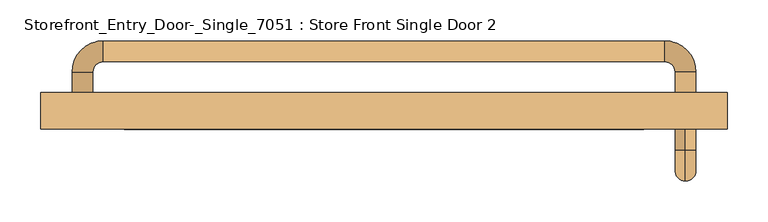
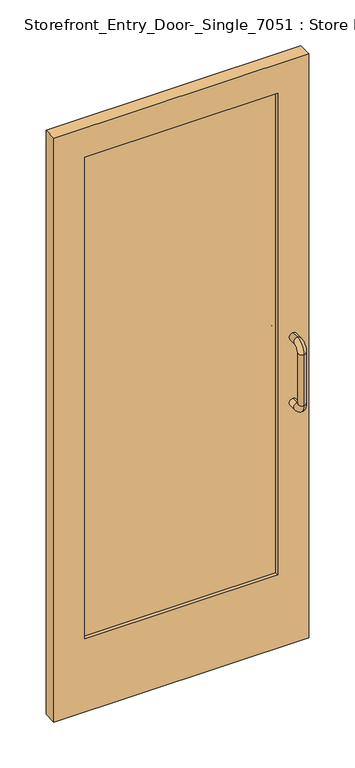
"""IFC4 building model written with IfcOpenShell, lengths in millimetres: door geometry, Storefront_Entry_Door-_Single_7051 : Store Front Single Door 2."""

import ifcopenshell
import ifcopenshell.guid

model = None  # the IFC model being written
_history = None  # IfcOwnerHistory: only IFC2X3 demands one
_inside = {}  # id of a spatial element -> (the spatial element, [elements in it])
_under = {}  # id of a project, library or spatial element -> (it, [spatial elements below it])
_declared = {}  # id of a project -> (the project, [libraries it declares])
_typed = {}  # id of a type object -> (the type object, [elements of that type])
_made_of = {}  # id of a material, layer set ... -> (it, [elements and type objects made of it])


def new_model(schema):
    """Start an empty IFC model of exactly this schema.

    Asked for "IFC4X3", IfcOpenShell would pick the latest addendum, in which some entities
    have other attributes; the version numbers below select the first issue.
    IFC2X3 requires an IfcOwnerHistory on every rooted entity: one is made here for all.
    """
    global model, _history
    if schema == "IFC4X3":
        model = ifcopenshell.file(schema_version=(4, 3, 0, 0))
    else:
        model = ifcopenshell.file(schema=schema)
    _inside.clear()
    _under.clear()
    _declared.clear()
    _typed.clear()
    _made_of.clear()
    _history = None
    if model.schema == "IFC2X3":
        org = make("IfcOrganization", Name="unknown")
        user = make(
            "IfcPersonAndOrganization",
            ThePerson=make("IfcPerson", FamilyName="unknown"),
            TheOrganization=org,
        )
        app = make(
            "IfcApplication",
            ApplicationDeveloper=org,
            Version="unknown",
            ApplicationFullName="unknown",
            ApplicationIdentifier="unknown",
        )
        _history = make(
            "IfcOwnerHistory",
            OwningUser=user,
            OwningApplication=app,
            ChangeAction="ADDED",
            CreationDate=0,
        )
    return model


def make(cls, **values):
    """One entity of the class cls with the attributes given. An attribute that is None is left unset."""
    return model.create_entity(
        cls, **{name: value for name, value in values.items() if value is not None}
    )


def rooted(cls, **values):
    """An entity with a GlobalId (a new one), such as an element, a storey or a relation."""
    return make(cls, GlobalId=ifcopenshell.guid.new(), OwnerHistory=_history, **values)


def si_unit(unit_type, name, prefix=None):
    """IfcSIUnit, for example si_unit("LENGTHUNIT", "METRE", prefix="MILLI")."""
    return make("IfcSIUnit", UnitType=unit_type, Prefix=prefix, Name=name)


def assignment(units):
    """IfcUnitAssignment: the units of a project."""
    return None if units is None else make("IfcUnitAssignment", Units=units)


def point(xyz):
    """IfcCartesianPoint."""
    return None if xyz is None else make("IfcCartesianPoint", Coordinates=xyz)


def direction(xyz):
    """IfcDirection."""
    return None if xyz is None else make("IfcDirection", DirectionRatios=xyz)


def frame(location, z_axis=None, x_axis=None):
    """IfcAxis2Placement3D, a coordinate frame: its origin and axes. An axis left out is left unset."""
    return make(
        "IfcAxis2Placement3D",
        Location=point(location),
        Axis=direction(z_axis),
        RefDirection=direction(x_axis),
    )


def origin():
    """The frame at (0, 0, 0) with its axes left unset."""
    return frame((0.0, 0.0, 0.0))


def place(relative_to, where):
    """IfcLocalPlacement: puts the frame where relative to a parent placement (None: the world)."""
    return make(
        "IfcLocalPlacement", PlacementRelTo=relative_to, RelativePlacement=where
    )


def context(
    kind, dimensions, precision=None, world=None, true_north=None, identifier=None
):
    """IfcGeometricRepresentationContext, for example the 3D "Model" context."""
    return make(
        "IfcGeometricRepresentationContext",
        ContextIdentifier=identifier,
        ContextType=kind,
        CoordinateSpaceDimension=dimensions,
        Precision=precision,
        WorldCoordinateSystem=world,
        TrueNorth=true_north,
    )


def project(units=None, contexts=None):
    """IfcProject with its units and contexts."""
    return rooted(
        "IfcProject",
        Name="project",
        RepresentationContexts=contexts,
        UnitsInContext=assignment(units),
    )


def spatial(cls, under=None, at=None, **own):
    """A site, building, storey or space (cls), placed at a placement, below another one or the project."""
    s = rooted(cls, ObjectPlacement=at, **own)
    if under is not None:
        _under.setdefault(under.id(), (under, []))[1].append(s)
    return s


def polyline(points):
    """IfcPolyline through the points."""
    return make("IfcPolyline", Points=[point(p) for p in points])


def circle_curve(where, radius):
    """IfcCircle in the frame where."""
    return make("IfcCircle", Position=where, Radius=radius)


def ellipse_curve(where, semi_axis1, semi_axis2):
    """IfcEllipse in the frame where."""
    return make(
        "IfcEllipse", Position=where, SemiAxis1=semi_axis1, SemiAxis2=semi_axis2
    )


def trimmed(basis, trim1, trim2, sense, master):
    """IfcTrimmedCurve: the piece of a basis curve between two trims."""
    return make(
        "IfcTrimmedCurve",
        BasisCurve=basis,
        Trim1=trim1,
        Trim2=trim2,
        SenseAgreement=sense,
        MasterRepresentation=master,
    )


def outline(outer, holes=None, kind="AREA"):
    """IfcArbitraryClosedProfileDef: a profile drawn as a closed curve; with holes, ...WithVoids."""
    if holes is None:
        return make("IfcArbitraryClosedProfileDef", ProfileType=kind, OuterCurve=outer)
    return make(
        "IfcArbitraryProfileDefWithVoids",
        ProfileType=kind,
        OuterCurve=outer,
        InnerCurves=holes,
    )


def extrude(swept, where, along, depth):
    """IfcExtrudedAreaSolid: the profile swept, set in the frame where, extruded along a direction by depth."""
    return make(
        "IfcExtrudedAreaSolid",
        SweptArea=swept,
        Position=where,
        ExtrudedDirection=direction(along),
        Depth=depth,
    )


def shape(context_of_items, identifier, shape_type, items):
    """IfcShapeRepresentation: the items that make up one representation, for example the "Body"."""
    return make(
        "IfcShapeRepresentation",
        ContextOfItems=context_of_items,
        RepresentationIdentifier=identifier,
        RepresentationType=shape_type,
        Items=items,
    )


def source(mapping_origin, context_of_items, identifier, shape_type, items):
    """IfcRepresentationMap: a shape defined once, which mapped items show again and again."""
    return make(
        "IfcRepresentationMap",
        MappingOrigin=mapping_origin,
        MappedRepresentation=shape(context_of_items, identifier, shape_type, items),
    )


def transform(
    local_origin,
    x_axis=None,
    y_axis=None,
    z_axis=None,
    scale=None,
    scale2=None,
    scale3=None,
    uniform=True,
):
    """IfcCartesianTransformationOperator3D, or its non-uniform kind. x_axis, y_axis, z_axis: its Axis1, 2, 3."""
    if uniform:
        return make(
            "IfcCartesianTransformationOperator3D",
            Axis1=direction(x_axis),
            Axis2=direction(y_axis),
            LocalOrigin=point(local_origin),
            Scale=scale,
            Axis3=direction(z_axis),
        )
    return make(
        "IfcCartesianTransformationOperator3DnonUniform",
        Axis1=direction(x_axis),
        Axis2=direction(y_axis),
        LocalOrigin=point(local_origin),
        Scale=scale,
        Axis3=direction(z_axis),
        Scale2=scale2,
        Scale3=scale3,
    )


def mapped(mapping_source, mapping_target):
    """IfcMappedItem: shows the shape of a source again, moved by a transform."""
    return make(
        "IfcMappedItem", MappingSource=mapping_source, MappingTarget=mapping_target
    )


def made_of(thing, what):
    """Note that an element or type object is made of a material, layer set ...; save() writes the relation."""
    if what is not None:
        _made_of.setdefault(what.id(), (what, []))[1].append(thing)
    return thing


def element(
    cls,
    number,
    at=None,
    inside=None,
    cuts=None,
    type_object=None,
    material=None,
    context=None,
    identifier="Body",
    shape_type=None,
    held_by="IfcProductDefinitionShape",
    body=None,
    shapes=None,
    **own,
):
    """One element of the class cls, such as IfcWall. Its Tag is "e" and its number.

    at: its placement. inside: the storey or other place that contains it. cuts: it is an
    opening in that element (IfcRelVoidsElement). A single representation is given by context,
    identifier, shape_type and body (its items); several are given by shapes. held_by: the class
    of the entity that holds the representations. save() writes the other relations.
    """
    e = rooted(cls, Tag="e%d" % number, ObjectPlacement=at, **own)
    if body is not None:
        shapes = [shape(context, identifier, shape_type, body)]
    if shapes is not None:
        e.Representation = make(held_by, Representations=shapes)
    if inside is not None:
        _inside.setdefault(inside.id(), (inside, []))[1].append(e)
    if cuts is not None:
        rooted(
            "IfcRelVoidsElement", RelatingBuildingElement=cuts, RelatedOpeningElement=e
        )
    if type_object is not None:
        _typed.setdefault(type_object.id(), (type_object, []))[1].append(e)
    return made_of(e, material)


def aggregate(whole, parts):
    """IfcRelAggregates: a whole, such as a stair, and the parts it consists of."""
    return rooted("IfcRelAggregates", RelatingObject=whole, RelatedObjects=parts)


def save(model, path):
    """Write the relations noted so far, then the file.

    IfcRelAggregates (storeys below a building ...), IfcRelContainedInSpatialStructure (elements
    in a storey), IfcRelDefinesByType, IfcRelAssociatesMaterial and IfcRelDeclares: one each for
    every whole, place, type object, material and project.
    """
    for whole, parts in _under.values():
        aggregate(whole, parts)
    for where, things in _inside.values():
        rooted(
            "IfcRelContainedInSpatialStructure",
            RelatedElements=things,
            RelatingStructure=where,
        )
    for kind, things in _typed.values():
        rooted("IfcRelDefinesByType", RelatedObjects=things, RelatingType=kind)
    for what, things in _made_of.values():
        rooted("IfcRelAssociatesMaterial", RelatedObjects=things, RelatingMaterial=what)
    for by, libraries in _declared.values():
        rooted("IfcRelDeclares", RelatingContext=by, RelatedDefinitions=libraries)
    model.write(path)


def plane_surface(at):
    """IfcPlane: the flat surface through the origin of the frame at, square to its z axis."""
    return make("IfcPlane", Position=at)


def cylinder_surface(at, radius):
    """IfcCylindricalSurface: all points at the distance radius from the z axis of the frame at."""
    return make("IfcCylindricalSurface", Position=at, Radius=radius)


def revolved_surface(curve, axis_point, axis_direction):
    """IfcSurfaceOfRevolution: the curve turned about the line through axis_point along axis_direction."""
    return make(
        "IfcSurfaceOfRevolution",
        SweptCurve=make("IfcArbitraryOpenProfileDef", ProfileType="CURVE", Curve=curve),
        AxisPosition=make("IfcAxis1Placement", Location=point(axis_point), Axis=direction(axis_direction)),
    )


def advanced_brep(points, edges, surfaces, faces):
    """IfcAdvancedBrep: a solid bounded by faces that lie on surfaces and meet in shared edges.

    An edge is (start, end): straight between two places in points (the first is 0);
    or (start, end, curve); or (start, end, curve, False) where it runs against its curve.
    A face is (place in surfaces, loops), or (place, loops, False) where it looks against
    its surface's normal. A loop lists edges by number (the first is 1), with a minus sign
    where the edge is run from its end to its start. The first loop is the outer one.
    """
    corners = [point(p) for p in points]
    vertices = [make("IfcVertexPoint", VertexGeometry=c) for c in corners]
    made = []
    for start, end, *more in edges:
        made.append(
            make(
                "IfcEdgeCurve",
                EdgeStart=vertices[start],
                EdgeEnd=vertices[end],
                EdgeGeometry=more[0] if more else make("IfcPolyline", Points=[corners[start], corners[end]]),
                SameSense=more[1] if len(more) > 1 else True,
            )
        )
    hull = []
    for where, loops, *sense in faces:
        bounds = []
        for j, loop in enumerate(loops):
            ring = [make("IfcOrientedEdge", EdgeElement=made[abs(k) - 1], Orientation=k > 0) for k in loop]
            bounds.append(
                make(
                    "IfcFaceOuterBound" if j == 0 else "IfcFaceBound",
                    Bound=make("IfcEdgeLoop", EdgeList=ring),
                    Orientation=True,
                )
            )
        hull.append(make("IfcAdvancedFace", Bounds=bounds, FaceSurface=surfaces[where], SameSense=sense[0] if sense else True))
    return make("IfcAdvancedBrep", Outer=make("IfcClosedShell", CfsFaces=hull))


def storefront_entry_door_single_7051_store_front_single_door_2_fbd616a1(model_context):
    return source(origin(), model_context, "Body", "SolidModel", [
        advanced_brep(
        [(368.3000002, -50.8, 1054.1), (368.3000002, -50.8, 1079.5), (368.3000002, -76.2, 1079.5), (368.3000002, -76.2, 1054.1), (368.3000002, -114.3, 1041.4), (368.3000002, -88.9, 1041.4), (368.3000002, -114.3, 863.6), (368.3000002, -88.9, 863.6), (368.3000002, -76.2, 825.5), (368.3000002, -76.2, 850.9), (368.3000002, -50.8, 850.9), (368.3000002, -50.8, 825.5)],
        [
            (0, 1, circle_curve(frame((368.3000002, -50.8, 1066.8), z_axis=(0.0, 1.0, 0.0), x_axis=(0.0, 0.0, 1.0)), 12.7)),
            (1, 0, circle_curve(frame((368.3000002, -50.8, 1066.8), z_axis=(0.0, 1.0, 0.0), x_axis=(0.0, 0.0, 1.0)), 12.7)),
            (1, 2),
            (2, 3, circle_curve(frame((368.3000002, -76.2, 1066.8), z_axis=(0.0, 1.0, 0.0), x_axis=(0.0, 0.0, 1.0)), 12.7)),
            (3, 0),
            (3, 2, circle_curve(frame((368.3000002, -76.2, 1066.8), z_axis=(0.0, 1.0, 0.0), x_axis=(0.0, 0.0, 1.0)), 12.7)),
            (4, 5, circle_curve(frame((368.3000002, -101.6, 1041.4), z_axis=(0.0, 0.0, 1.0), x_axis=(0.0, -1.0, 0.0)), 12.7)),
            (5, 3, circle_curve(frame((368.3000002, -76.2, 1041.4), z_axis=(-1.0, 0.0, 0.0), x_axis=(0.0, 0.0, 1.0)), 12.7)),
            (2, 4, circle_curve(frame((368.3000002, -76.2, 1041.4), z_axis=(1.0, 0.0, 0.0), x_axis=(0.0, 0.0, 1.0)), 38.1)),
            (5, 4, circle_curve(frame((368.3000002, -101.6, 1041.4), z_axis=(0.0, 0.0, 1.0), x_axis=(0.0, -1.0, 0.0)), 12.7)),
            (4, 6),
            (6, 7, circle_curve(frame((368.3000002, -101.6, 863.6), z_axis=(0.0, 0.0, 1.0), x_axis=(0.0, -1.0, 0.0)), 12.7)),
            (7, 5),
            (7, 6, circle_curve(frame((368.3000002, -101.6, 863.6), z_axis=(0.0, 0.0, 1.0), x_axis=(0.0, -1.0, 0.0)), 12.7)),
            (8, 9, circle_curve(frame((368.3000002, -76.2, 838.2), z_axis=(0.0, -1.0, 0.0), x_axis=(0.0, 0.0, -1.0)), 12.7)),
            (9, 7, circle_curve(frame((368.3000002, -76.2, 863.6), z_axis=(-1.0, 0.0, 0.0), x_axis=(0.0, -1.0, 0.0)), 12.7)),
            (6, 8, circle_curve(frame((368.3000002, -76.2, 863.6), z_axis=(1.0, 0.0, 0.0), x_axis=(0.0, -1.0, 0.0)), 38.1)),
            (9, 8, circle_curve(frame((368.3000002, -76.2, 838.2), z_axis=(0.0, -1.0, 0.0), x_axis=(0.0, 0.0, -1.0)), 12.7)),
            (10, 11, circle_curve(frame((368.3000002, -50.8, 838.2), z_axis=(0.0, 1.0, 0.0), x_axis=(0.0, 0.0, -1.0)), 12.7)),
            (11, 10, circle_curve(frame((368.3000002, -50.8, 838.2), z_axis=(0.0, 1.0, 0.0), x_axis=(0.0, 0.0, -1.0)), 12.7)),
            (8, 11),
            (10, 9),
        ],
        [
            plane_surface(frame((368.3000002, -50.8, 1066.8), z_axis=(0.0, 1.0, 0.0), x_axis=(1.0, 0.0, 0.0))),
            cylinder_surface(frame((368.3000002, -50.8, 1066.8), z_axis=(0.0, 1.0, 0.0), x_axis=(0.0, 0.0, 1.0)), 12.7),
            revolved_surface(trimmed(ellipse_curve(frame((368.3000002, -76.2, 1066.8), z_axis=(0.0, -1.0, 0.0), x_axis=(0.0, 0.0, 1.0)), 12.7, 12.7), [point((368.3000002, -76.2, 1054.1))], [point((368.3000002, -76.2, 1079.5))], True, "CARTESIAN"), (368.3000002, -76.2, 1041.4), (-1.0, 0.0, 0.0)),
            revolved_surface(trimmed(ellipse_curve(frame((368.3000002, -76.2, 1066.8), z_axis=(0.0, -1.0, 0.0), x_axis=(0.0, 0.0, 1.0)), 12.7, 12.7), [point((368.3000002, -76.2, 1079.5))], [point((368.3000002, -76.2, 1054.1))], True, "CARTESIAN"), (368.3000002, -76.2, 1041.4), (-1.0, 0.0, 0.0)),
            cylinder_surface(frame((368.3000002, -101.6, 1041.4), z_axis=(0.0, 0.0, 1.0), x_axis=(0.0, -1.0, 0.0)), 12.7),
            revolved_surface(trimmed(ellipse_curve(frame((368.3000002, -101.6, 863.6), z_axis=(0.0, 0.0, -1.0), x_axis=(0.0, -1.0, 0.0)), 12.7, 12.7), [point((368.3000002, -88.9, 863.6))], [point((368.3000002, -114.3, 863.6))], True, "CARTESIAN"), (368.3000002, -76.2, 863.6), (-1.0, 0.0, 0.0)),
            revolved_surface(trimmed(ellipse_curve(frame((368.3000002, -101.6, 863.6), z_axis=(0.0, 0.0, -1.0), x_axis=(0.0, -1.0, 0.0)), 12.7, 12.7), [point((368.3000002, -114.3, 863.6))], [point((368.3000002, -88.9, 863.6))], True, "CARTESIAN"), (368.3000002, -76.2, 863.6), (-1.0, 0.0, 0.0)),
            plane_surface(frame((368.3000002, -50.8, 838.2), z_axis=(0.0, 1.0, 0.0), x_axis=(1.0, 0.0, 0.0))),
            cylinder_surface(frame((368.3000002, -76.2, 838.2), z_axis=(0.0, -1.0, 0.0), x_axis=(0.0, 0.0, -1.0)), 12.7),
        ],
        [
            (0, [[1, 2]]),
            (1, [[3, 4, 5, -2]]),
            (1, [[-5, 6, -3, -1]]),
            (2, [[7, 8, -4, 9]]),
            (3, [[10, -9, -6, -8]]),
            (4, [[11, 12, 13, -7]]),
            (4, [[-13, 14, -11, -10]]),
            (5, [[15, 16, -12, 17]]),
            (6, [[18, -17, -14, -16]]),
            (7, [[19, 20]]),
            (8, [[21, -19, 22, -15]]),
            (8, [[-22, -20, -21, -18]]),
        ],
    ),
        advanced_brep(
        [(355.6000002, -6.35, 1066.8), (381.0000002, -6.35, 1066.8), (381.0000002, 19.05, 1066.8), (355.6000002, 19.05, 1066.8), (342.9000002, 57.15, 1066.8), (342.9000002, 31.75, 1066.8), (-342.9000002, 57.15, 1066.8), (-342.9000002, 31.75, 1066.8), (-381.0000002, 19.05, 1066.8), (-355.6000002, 19.05, 1066.8), (-355.6000002, -6.35, 1066.8), (-381.0000002, -6.35, 1066.8)],
        [
            (0, 1, circle_curve(frame((368.3000002, -6.35, 1066.8), z_axis=(0.0, -1.0, 0.0), x_axis=(1.0, 0.0, 0.0)), 12.7)),
            (1, 0, circle_curve(frame((368.3000002, -6.35, 1066.8), z_axis=(0.0, -1.0, 0.0), x_axis=(1.0, 0.0, 0.0)), 12.7)),
            (1, 2),
            (2, 3, circle_curve(frame((368.3000002, 19.05, 1066.8), z_axis=(0.0, -1.0, 0.0), x_axis=(1.0, 0.0, 0.0)), 12.7)),
            (3, 0),
            (3, 2, circle_curve(frame((368.3000002, 19.05, 1066.8), z_axis=(0.0, -1.0, 0.0), x_axis=(1.0, 0.0, 0.0)), 12.7)),
            (4, 5, circle_curve(frame((342.9000002, 44.45, 1066.8), z_axis=(1.0, 0.0, 0.0), x_axis=(0.0, 1.0, 0.0)), 12.7)),
            (5, 3, circle_curve(frame((342.9000002, 19.05, 1066.8), z_axis=(0.0, 0.0, -1.0), x_axis=(1.0, 0.0, 0.0)), 12.7)),
            (2, 4, circle_curve(frame((342.9000002, 19.05, 1066.8), z_axis=(0.0, 0.0, 1.0), x_axis=(1.0, 0.0, 0.0)), 38.1)),
            (5, 4, circle_curve(frame((342.9000002, 44.45, 1066.8), z_axis=(1.0, 0.0, 0.0), x_axis=(0.0, 1.0, 0.0)), 12.7)),
            (4, 6),
            (6, 7, circle_curve(frame((-342.9000002, 44.45, 1066.8), z_axis=(1.0, 0.0, 0.0), x_axis=(0.0, 1.0, 0.0)), 12.7)),
            (7, 5),
            (7, 6, circle_curve(frame((-342.9000002, 44.45, 1066.8), z_axis=(1.0, 0.0, 0.0), x_axis=(0.0, 1.0, 0.0)), 12.7)),
            (8, 9, circle_curve(frame((-368.3000002, 19.05, 1066.8), z_axis=(0.0, 1.0, 0.0), x_axis=(-1.0, 0.0, 0.0)), 12.7)),
            (9, 7, circle_curve(frame((-342.9000002, 19.05, 1066.8), z_axis=(0.0, 0.0, -1.0), x_axis=(0.0, 1.0, 0.0)), 12.7)),
            (6, 8, circle_curve(frame((-342.9000002, 19.05, 1066.8), z_axis=(0.0, 0.0, 1.0), x_axis=(0.0, 1.0, 0.0)), 38.1)),
            (9, 8, circle_curve(frame((-368.3000002, 19.05, 1066.8), z_axis=(0.0, 1.0, 0.0), x_axis=(-1.0, 0.0, 0.0)), 12.7)),
            (10, 11, circle_curve(frame((-368.3000002, -6.35, 1066.8), z_axis=(0.0, -1.0, 0.0), x_axis=(-1.0, 0.0, 0.0)), 12.7)),
            (11, 10, circle_curve(frame((-368.3000002, -6.35, 1066.8), z_axis=(0.0, -1.0, 0.0), x_axis=(-1.0, 0.0, 0.0)), 12.7)),
            (8, 11),
            (10, 9),
        ],
        [
            plane_surface(frame((368.3000002, -6.35, 1066.8), z_axis=(0.0, -1.0, 0.0), x_axis=(0.0, 0.0, 1.0))),
            cylinder_surface(frame((368.3000002, -6.35, 1066.8), z_axis=(0.0, -1.0, 0.0), x_axis=(1.0, 0.0, 0.0)), 12.7),
            revolved_surface(trimmed(ellipse_curve(frame((368.3000002, 19.05, 1066.8), z_axis=(0.0, 1.0, 0.0), x_axis=(1.0, 0.0, 0.0)), 12.7, 12.7), [point((355.6000002, 19.05, 1066.8))], [point((381.0000002, 19.05, 1066.8))], True, "CARTESIAN"), (342.9000002, 19.05, 1066.8), (0.0, 0.0, -1.0)),
            revolved_surface(trimmed(ellipse_curve(frame((368.3000002, 19.05, 1066.8), z_axis=(0.0, 1.0, 0.0), x_axis=(1.0, 0.0, 0.0)), 12.7, 12.7), [point((381.0000002, 19.05, 1066.8))], [point((355.6000002, 19.05, 1066.8))], True, "CARTESIAN"), (342.9000002, 19.05, 1066.8), (0.0, 0.0, -1.0)),
            cylinder_surface(frame((342.9000002, 44.45, 1066.8), z_axis=(1.0, 0.0, 0.0), x_axis=(0.0, 1.0, 0.0)), 12.7),
            revolved_surface(trimmed(ellipse_curve(frame((-342.9000002, 44.45, 1066.8), z_axis=(-1.0, 0.0, 0.0), x_axis=(0.0, 1.0, 0.0)), 12.7, 12.7), [point((-342.9000002, 31.75, 1066.8))], [point((-342.9000002, 57.15, 1066.8))], True, "CARTESIAN"), (-342.9000002, 19.05, 1066.8), (0.0, 0.0, -1.0)),
            revolved_surface(trimmed(ellipse_curve(frame((-342.9000002, 44.45, 1066.8), z_axis=(-1.0, 0.0, 0.0), x_axis=(0.0, 1.0, 0.0)), 12.7, 12.7), [point((-342.9000002, 57.15, 1066.8))], [point((-342.9000002, 31.75, 1066.8))], True, "CARTESIAN"), (-342.9000002, 19.05, 1066.8), (0.0, 0.0, -1.0)),
            plane_surface(frame((-368.3000002, -6.35, 1066.8), z_axis=(0.0, -1.0, 0.0), x_axis=(0.0, 0.0, 1.0))),
            cylinder_surface(frame((-368.3000002, 19.05, 1066.8), z_axis=(0.0, 1.0, 0.0), x_axis=(-1.0, 0.0, 0.0)), 12.7),
        ],
        [
            (0, [[1, 2]]),
            (1, [[3, 4, 5, -2]]),
            (1, [[-5, 6, -3, -1]]),
            (2, [[7, 8, -4, 9]]),
            (3, [[10, -9, -6, -8]]),
            (4, [[11, 12, 13, -7]]),
            (4, [[-13, 14, -11, -10]]),
            (5, [[15, 16, -12, 17]]),
            (6, [[18, -17, -14, -16]]),
            (7, [[19, 20]]),
            (8, [[21, -19, 22, -15]]),
            (8, [[-22, -20, -21, -18]]),
        ],
    ),
        extrude(outline(polyline([(317.5000002, -19.05), (317.5000002, -38.1), (-317.5000002, -38.1), (-317.5000002, -19.05), (317.5000002, -19.05)])), frame((0.0, 0.0, 254.0), z_axis=(0.0, 0.0, 1.0), x_axis=(1.0, 0.0, 0.0)), (0.0, 0.0, 1.0), 1676.4),
        extrude(outline(polyline([(2032.0, 419.1000002), (2032.0, -419.1000002), (0.0, -419.1000002), (0.0, 419.1000002), (2032.0, 419.1000002)]), holes=[polyline([(1930.4, -317.5000002), (1930.4, 317.5000002), (254.0, 317.5000002), (254.0, -317.5000002), (1930.4, -317.5000002)])]), frame((0.0, -50.8, 0.0), z_axis=(0.0, 1.0, 0.0), x_axis=(0.0, 0.0, 1.0)), (0.0, 0.0, 1.0), 44.45),
    ])


if __name__ == "__main__":
    model = new_model("IFC4")
    model_context = context("Model", 3, world=origin())
    ifc_project = project(units=[si_unit("LENGTHUNIT", "METRE", prefix="MILLI")], contexts=[model_context])
    site = spatial("IfcSite", under=ifc_project)
    building = spatial("IfcBuilding", under=site)
    placement = place(None, origin())
    storefront_entry_door_single_7051_store_front_single_door_2_shape = storefront_entry_door_single_7051_store_front_single_door_2_fbd616a1(model_context)
    element("IfcDoor", 1, ObjectType="Storefront_Entry_Door-_Single_7051 : Store Front Single Door 2", at=placement, inside=building, context=model_context, shape_type="MappedRepresentation", body=[
        mapped(storefront_entry_door_single_7051_store_front_single_door_2_shape, transform((0.0, 0.0, 0.0), x_axis=(1.0, 0.0, 0.0), y_axis=(0.0, 1.0, 0.0), z_axis=(0.0, 0.0, 1.0))),
    ])
    save(model, "model.ifc")

# Revit data of these elements
# Type "Storefront_Entry_Door-_Single_7051 : Store Front Single Door 2"
#   Type Mark = "26"
#   Assembly Code = "B2030110"
#   Analytic Construction = "<None>"
#   Top Rail = 0' - 4"
#   Side Rail = 0' - 4"
#   Reporting Width [instance default] = 4' - 2"
#   Rail Height AFF = 3' - 6"
#   Offset = 0' - 2"
#   Door Width [instance default] = 4' - 2"
#   Bottom Rail Width = 0' - 10"
#   Material = accent 1
#   Glazing Material = Glass
#   Function = (empty or 0)
# Element 1 (IfcDoor, "Storefront_Entry_Door-_Single_7051 : Store Front Single Door 2")
#   Reporting Width = 2' - 9"
#   Door Width = 2' - 9"
#   Materials on its faces: "accent 1", "Glass"
# Materials
#   "accent 1": class "Generic", colour RGB 92 104 51, transparency 0, Cost = 0
#   "Glass": class "Glass", colour RGB 236 240 239, transparency 0.85, Description = "Soda Lime Glass", Cost = 0
